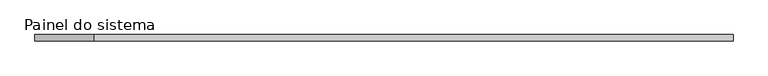
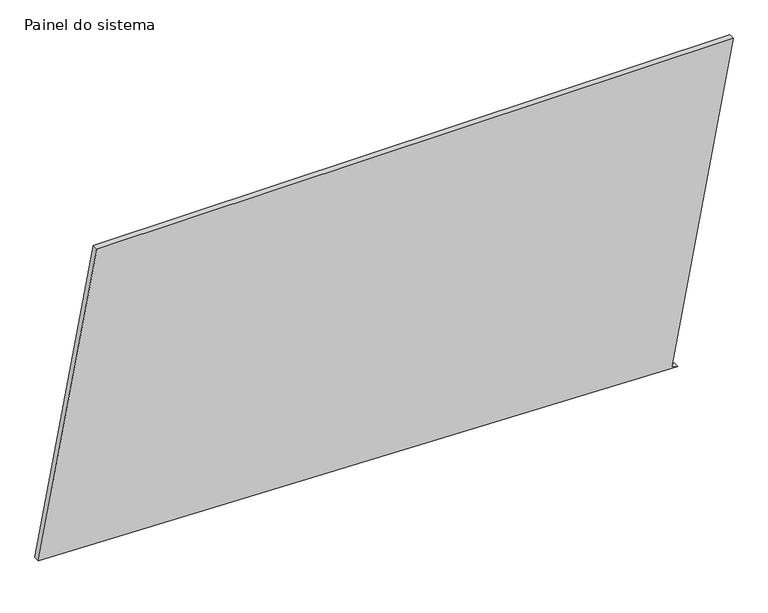
"""IFC4 building model written with IfcOpenShell, lengths in millimetres: plate geometry, Painel do sistema : Envidraçado."""

import ifcopenshell
import ifcopenshell.guid

model = None  # the IFC model being written
_history = None  # IfcOwnerHistory: only IFC2X3 demands one
_inside = {}  # id of a spatial element -> (the spatial element, [elements in it])
_under = {}  # id of a project, library or spatial element -> (it, [spatial elements below it])
_declared = {}  # id of a project -> (the project, [libraries it declares])
_typed = {}  # id of a type object -> (the type object, [elements of that type])
_made_of = {}  # id of a material, layer set ... -> (it, [elements and type objects made of it])


def new_model(schema):
    """Start an empty IFC model of exactly this schema.

    Asked for "IFC4X3", IfcOpenShell would pick the latest addendum, in which some entities
    have other attributes; the version numbers below select the first issue.
    IFC2X3 requires an IfcOwnerHistory on every rooted entity: one is made here for all.
    """
    global model, _history
    if schema == "IFC4X3":
        model = ifcopenshell.file(schema_version=(4, 3, 0, 0))
    else:
        model = ifcopenshell.file(schema=schema)
    _inside.clear()
    _under.clear()
    _declared.clear()
    _typed.clear()
    _made_of.clear()
    _history = None
    if model.schema == "IFC2X3":
        org = make("IfcOrganization", Name="unknown")
        user = make(
            "IfcPersonAndOrganization",
            ThePerson=make("IfcPerson", FamilyName="unknown"),
            TheOrganization=org,
        )
        app = make(
            "IfcApplication",
            ApplicationDeveloper=org,
            Version="unknown",
            ApplicationFullName="unknown",
            ApplicationIdentifier="unknown",
        )
        _history = make(
            "IfcOwnerHistory",
            OwningUser=user,
            OwningApplication=app,
            ChangeAction="ADDED",
            CreationDate=0,
        )
    return model


def make(cls, **values):
    """One entity of the class cls with the attributes given. An attribute that is None is left unset."""
    return model.create_entity(
        cls, **{name: value for name, value in values.items() if value is not None}
    )


def rooted(cls, **values):
    """An entity with a GlobalId (a new one), such as an element, a storey or a relation."""
    return make(cls, GlobalId=ifcopenshell.guid.new(), OwnerHistory=_history, **values)


def si_unit(unit_type, name, prefix=None):
    """IfcSIUnit, for example si_unit("LENGTHUNIT", "METRE", prefix="MILLI")."""
    return make("IfcSIUnit", UnitType=unit_type, Prefix=prefix, Name=name)


def assignment(units):
    """IfcUnitAssignment: the units of a project."""
    return None if units is None else make("IfcUnitAssignment", Units=units)


def point(xyz):
    """IfcCartesianPoint."""
    return None if xyz is None else make("IfcCartesianPoint", Coordinates=xyz)


def direction(xyz):
    """IfcDirection."""
    return None if xyz is None else make("IfcDirection", DirectionRatios=xyz)


def frame(location, z_axis=None, x_axis=None):
    """IfcAxis2Placement3D, a coordinate frame: its origin and axes. An axis left out is left unset."""
    return make(
        "IfcAxis2Placement3D",
        Location=point(location),
        Axis=direction(z_axis),
        RefDirection=direction(x_axis),
    )


def origin():
    """The frame at (0, 0, 0) with its axes left unset."""
    return frame((0.0, 0.0, 0.0))


def place(relative_to, where):
    """IfcLocalPlacement: puts the frame where relative to a parent placement (None: the world)."""
    return make(
        "IfcLocalPlacement", PlacementRelTo=relative_to, RelativePlacement=where
    )


def context(
    kind, dimensions, precision=None, world=None, true_north=None, identifier=None
):
    """IfcGeometricRepresentationContext, for example the 3D "Model" context."""
    return make(
        "IfcGeometricRepresentationContext",
        ContextIdentifier=identifier,
        ContextType=kind,
        CoordinateSpaceDimension=dimensions,
        Precision=precision,
        WorldCoordinateSystem=world,
        TrueNorth=true_north,
    )


def project(units=None, contexts=None):
    """IfcProject with its units and contexts."""
    return rooted(
        "IfcProject",
        Name="project",
        RepresentationContexts=contexts,
        UnitsInContext=assignment(units),
    )


def spatial(cls, under=None, at=None, **own):
    """A site, building, storey or space (cls), placed at a placement, below another one or the project."""
    s = rooted(cls, ObjectPlacement=at, **own)
    if under is not None:
        _under.setdefault(under.id(), (under, []))[1].append(s)
    return s


def polyline(points):
    """IfcPolyline through the points."""
    return make("IfcPolyline", Points=[point(p) for p in points])


def outline(outer, holes=None, kind="AREA"):
    """IfcArbitraryClosedProfileDef: a profile drawn as a closed curve; with holes, ...WithVoids."""
    if holes is None:
        return make("IfcArbitraryClosedProfileDef", ProfileType=kind, OuterCurve=outer)
    return make(
        "IfcArbitraryProfileDefWithVoids",
        ProfileType=kind,
        OuterCurve=outer,
        InnerCurves=holes,
    )


def extrude(swept, where, along, depth):
    """IfcExtrudedAreaSolid: the profile swept, set in the frame where, extruded along a direction by depth."""
    return make(
        "IfcExtrudedAreaSolid",
        SweptArea=swept,
        Position=where,
        ExtrudedDirection=direction(along),
        Depth=depth,
    )


def shape(context_of_items, identifier, shape_type, items):
    """IfcShapeRepresentation: the items that make up one representation, for example the "Body"."""
    return make(
        "IfcShapeRepresentation",
        ContextOfItems=context_of_items,
        RepresentationIdentifier=identifier,
        RepresentationType=shape_type,
        Items=items,
    )


def source(mapping_origin, context_of_items, identifier, shape_type, items):
    """IfcRepresentationMap: a shape defined once, which mapped items show again and again."""
    return make(
        "IfcRepresentationMap",
        MappingOrigin=mapping_origin,
        MappedRepresentation=shape(context_of_items, identifier, shape_type, items),
    )


def transform(
    local_origin,
    x_axis=None,
    y_axis=None,
    z_axis=None,
    scale=None,
    scale2=None,
    scale3=None,
    uniform=True,
):
    """IfcCartesianTransformationOperator3D, or its non-uniform kind. x_axis, y_axis, z_axis: its Axis1, 2, 3."""
    if uniform:
        return make(
            "IfcCartesianTransformationOperator3D",
            Axis1=direction(x_axis),
            Axis2=direction(y_axis),
            LocalOrigin=point(local_origin),
            Scale=scale,
            Axis3=direction(z_axis),
        )
    return make(
        "IfcCartesianTransformationOperator3DnonUniform",
        Axis1=direction(x_axis),
        Axis2=direction(y_axis),
        LocalOrigin=point(local_origin),
        Scale=scale,
        Axis3=direction(z_axis),
        Scale2=scale2,
        Scale3=scale3,
    )


def mapped(mapping_source, mapping_target):
    """IfcMappedItem: shows the shape of a source again, moved by a transform."""
    return make(
        "IfcMappedItem", MappingSource=mapping_source, MappingTarget=mapping_target
    )


def made_of(thing, what):
    """Note that an element or type object is made of a material, layer set ...; save() writes the relation."""
    if what is not None:
        _made_of.setdefault(what.id(), (what, []))[1].append(thing)
    return thing


def element(
    cls,
    number,
    at=None,
    inside=None,
    cuts=None,
    type_object=None,
    material=None,
    context=None,
    identifier="Body",
    shape_type=None,
    held_by="IfcProductDefinitionShape",
    body=None,
    shapes=None,
    **own,
):
    """One element of the class cls, such as IfcWall. Its Tag is "e" and its number.

    at: its placement. inside: the storey or other place that contains it. cuts: it is an
    opening in that element (IfcRelVoidsElement). A single representation is given by context,
    identifier, shape_type and body (its items); several are given by shapes. held_by: the class
    of the entity that holds the representations. save() writes the other relations.
    """
    e = rooted(cls, Tag="e%d" % number, ObjectPlacement=at, **own)
    if body is not None:
        shapes = [shape(context, identifier, shape_type, body)]
    if shapes is not None:
        e.Representation = make(held_by, Representations=shapes)
    if inside is not None:
        _inside.setdefault(inside.id(), (inside, []))[1].append(e)
    if cuts is not None:
        rooted(
            "IfcRelVoidsElement", RelatingBuildingElement=cuts, RelatedOpeningElement=e
        )
    if type_object is not None:
        _typed.setdefault(type_object.id(), (type_object, []))[1].append(e)
    return made_of(e, material)


def aggregate(whole, parts):
    """IfcRelAggregates: a whole, such as a stair, and the parts it consists of."""
    return rooted("IfcRelAggregates", RelatingObject=whole, RelatedObjects=parts)


def save(model, path):
    """Write the relations noted so far, then the file.

    IfcRelAggregates (storeys below a building ...), IfcRelContainedInSpatialStructure (elements
    in a storey), IfcRelDefinesByType, IfcRelAssociatesMaterial and IfcRelDeclares: one each for
    every whole, place, type object, material and project.
    """
    for whole, parts in _under.values():
        aggregate(whole, parts)
    for where, things in _inside.values():
        rooted(
            "IfcRelContainedInSpatialStructure",
            RelatedElements=things,
            RelatingStructure=where,
        )
    for kind, things in _typed.values():
        rooted("IfcRelDefinesByType", RelatedObjects=things, RelatingType=kind)
    for what, things in _made_of.values():
        rooted("IfcRelAssociatesMaterial", RelatedObjects=things, RelatingMaterial=what)
    for by, libraries in _declared.values():
        rooted("IfcRelDeclares", RelatingContext=by, RelatedDefinitions=libraries)
    model.write(path)


def painel_do_sistema_a3bbbb36(model_context):
    return source(origin(), model_context, "Body", "SweptSolid", [
        extrude(outline(polyline([(0.0, 1189.1008089), (4.6288169, 1164.5330647), (1334.1499799, 1415.0285915), (1334.1499799, -1177.4244786), (73.0508277, -1415.0285915), (0.0, 1189.1008089)])), frame((0.0, 24.5, 0.0), z_axis=(0.0, 1.0, 0.0), x_axis=(0.0, 0.0, 1.0)), (0.0, 0.0, 1.0), 25.0),
    ])


if __name__ == "__main__":
    model = new_model("IFC4")
    model_context = context("Model", 3, world=origin())
    ifc_project = project(units=[si_unit("LENGTHUNIT", "METRE", prefix="MILLI")], contexts=[model_context])
    site = spatial("IfcSite", under=ifc_project)
    building = spatial("IfcBuilding", under=site)
    placement = place(None, origin())
    painel_do_sistema_shape = painel_do_sistema_a3bbbb36(model_context)
    element("IfcPlate", 1, ObjectType="Painel do sistema : Envidraçado", at=placement, inside=building, context=model_context, shape_type="MappedRepresentation", body=[
        mapped(painel_do_sistema_shape, transform((0.0, 0.0, 0.0), x_axis=(1.0, 0.0, 0.0), y_axis=(0.0, 1.0, 0.0), z_axis=(0.0, 0.0, 1.0))),
    ])
    save(model, "model.ifc")

# Revit data of these elements
# Type "Painel do sistema : Envidraçado"
#   Construction Type Id = "GSP4R"
#   Analytic Construction = "Vidraça única Pilkington 1/8 pol"
#   Visual Light Transmittance = 0.9
#   Solar Heat Gain Coefficient = 0.86
#   Heat Transfer Coefficient (U) = 6.7069 W/(m²·K)
# Element 1 (IfcPlate, "Painel do sistema : Envidraçado")
#   Materials on its faces: "Vidro"
# Materials
#   "Vidro": class "Vidro", colour RGB 0 128 192, transparency 0.9, Description = "Vidro de sílica", Cost = 0
